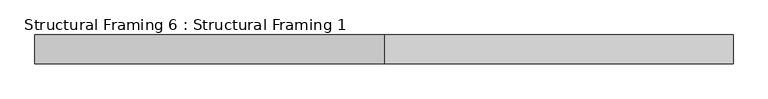
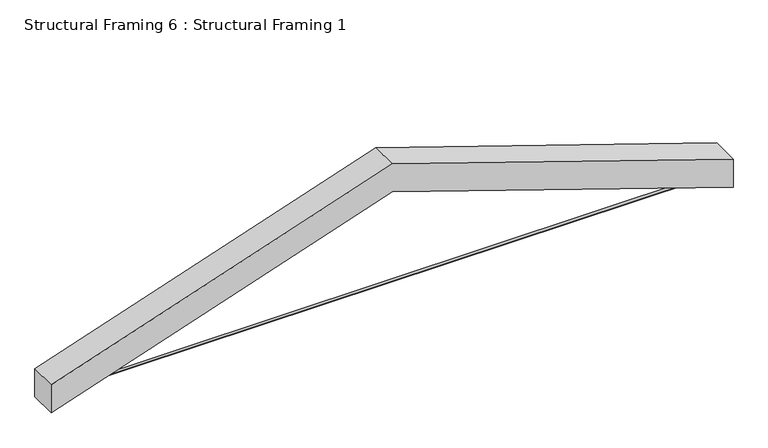
"""IFC4 building model written with IfcOpenShell, lengths in millimetres: beam geometry, Structural Framing 6 : Structural Framing 1."""

from ifc_helpers import new_model, si_unit, point, frame, frame_2d, origin, place, context, project, spatial, polyline, circle_curve, trimmed, segment, composite_curve, outline, extrude, source, transform, mapped, element, save


def structural_framing_6_structural_framing_1_610939d9(model_context):
    return source(origin(), model_context, "Body", "SweptSolid", [
        extrude(outline(composite_curve([segment(trimmed(circle_curve(frame_2d((-3484.8884634, 4984.3019529)), 6.35), [point((-3478.5384634, 4984.3019529))], [point((-3491.2384634, 4984.3019529))], False, "CARTESIAN"), True, "CONTINUOUS"), segment(trimmed(circle_curve(frame_2d((-3484.8884634, 4984.3019529)), 6.35), [point((-3491.2384634, 4984.3019529))], [point((-3478.5384634, 4984.3019529))], False, "CARTESIAN"), True, "CONTINUOUS")], self_intersect=False)), frame((19888.9870052, 0.0, 0.0), z_axis=(1.0, 0.0, 0.0), x_axis=(0.0, 1.0, 0.0)), (0.0, 0.0, 1.0), 3111.5),
        extrude(outline(polyline([(5652.475838, 21444.7370052), (5084.8528105, 19749.2870052), (4937.5315162, 19749.2870052), (5505.1545437, 21444.7370052), (4937.5315162, 23140.1870052), (5084.8528105, 23140.1870052), (5652.475838, 21444.7370052)])), frame((0.0, -3554.7384634, 0.0), z_axis=(0.0, 1.0, 0.0), x_axis=(0.0, 0.0, 1.0)), (0.0, 0.0, 1.0), 139.7),
    ])


if __name__ == "__main__":
    model = new_model("IFC4")
    model_context = context("Model", 3, world=origin())
    ifc_project = project(units=[si_unit("LENGTHUNIT", "METRE", prefix="MILLI")], contexts=[model_context])
    site = spatial("IfcSite", under=ifc_project)
    building = spatial("IfcBuilding", under=site)
    placement = place(None, origin())
    structural_framing_6_structural_framing_1_shape = structural_framing_6_structural_framing_1_610939d9(model_context)
    element("IfcBeam", 1, ObjectType="Structural Framing 6 : Structural Framing 1", at=placement, inside=building, context=model_context, shape_type="MappedRepresentation", body=[
        mapped(structural_framing_6_structural_framing_1_shape, transform((0.0, 0.0, 0.0), x_axis=(1.0, 0.0, 0.0), y_axis=(0.0, 1.0, 0.0), z_axis=(0.0, 0.0, 1.0))),
    ])
    save(model, "model.ifc")

# Revit data of these elements
# Element 1 (IfcBeam, "Structural Framing 6 : Structural Framing 1")
#   Materials on its faces: "GLULAM TRUSS W/ CUSTOM GUSSET PLATES", "COLLAR TIE: 1/2\" GALV. ROD"
# Materials
#   "GLULAM TRUSS W/ CUSTOM GUSSET PLATES": class "Generic", colour RGB 206 153 90, transparency 0, Cost = 0
#   "COLLAR TIE: 1/2\" GALV. ROD": class "Generic", colour RGB 49 49 49, transparency 0, Cost = 0
